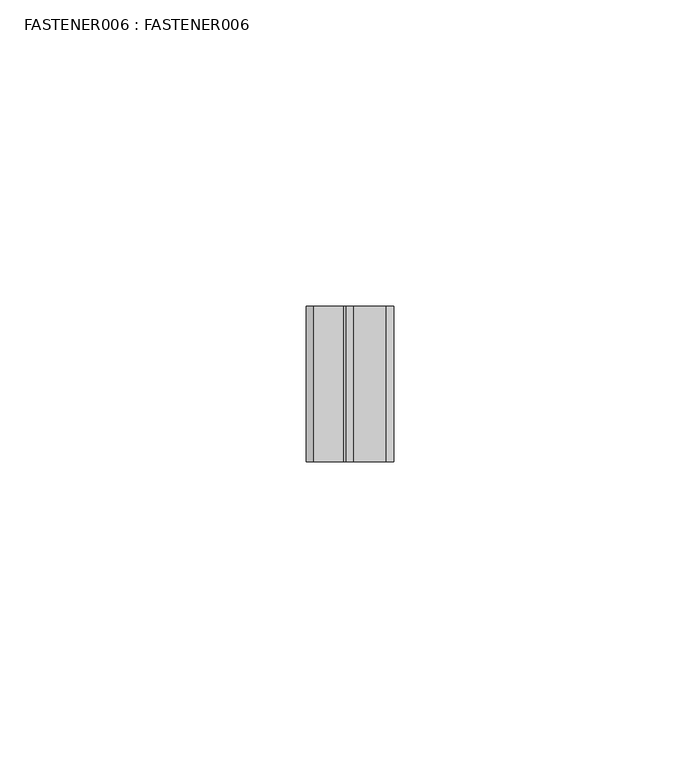
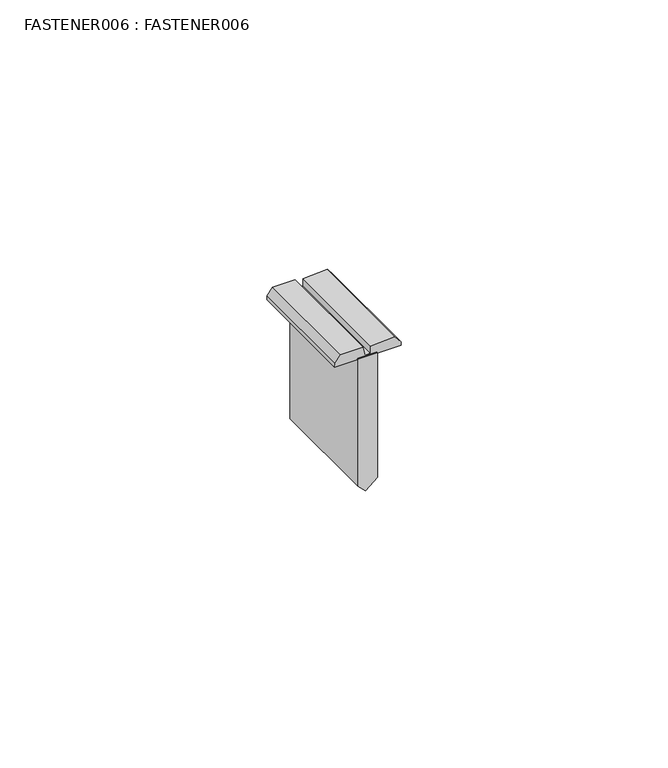
"""IFC4 building model written with IfcOpenShell, lengths in millimetres: proxy geometry, FASTENER006 : FASTENER006."""

from ifc_helpers import new_model, si_unit, frame, origin, place, context, project, spatial, polyline, outline, extrude, source, transform, mapped, element, save


def fastener006_fastener006_f031ca55(model_context):
    return source(origin(), model_context, "Body", "SweptSolid", [
        extrude(outline(polyline([(42577.1576024, 5870.6890035), (42548.1988623, 5870.6890035), (42546.5833096, 5872.3460181), (42548.7638676, 5874.895922), (42577.1576024, 5874.895922), (42577.1576024, 5870.6890035)])), frame((0.0, -1078.2906574, 0.0), z_axis=(0.0, 1.0, 0.0), x_axis=(0.0, 0.0, 1.0)), (0.0, 0.0, 1.0), 25.4),
        extrude(outline(polyline([(42577.1576024, 5879.9417891), (42577.9674245, 5879.9417891), (42579.5612959, 5878.7030871), (42579.1650604, 5873.4174049), (42577.5756297, 5873.4174049), (42577.5756297, 5872.1703), (42579.587761, 5871.7740645), (42579.587761, 5866.8949826), (42577.9938896, 5865.6562805), (42577.1576024, 5865.6454839), (42577.1576024, 5879.9417891)])), frame((0.0, -1078.2906574, 0.0), z_axis=(0.0, 1.0, 0.0), x_axis=(0.0, 0.0, 1.0)), (0.0, 0.0, 1.0), 25.4),
    ])


if __name__ == "__main__":
    model = new_model("IFC4")
    model_context = context("Model", 3, world=origin())
    ifc_project = project(units=[si_unit("LENGTHUNIT", "METRE", prefix="MILLI")], contexts=[model_context])
    site = spatial("IfcSite", under=ifc_project)
    building = spatial("IfcBuilding", under=site)
    placement = place(None, origin())
    fastener006_fastener006_shape = fastener006_fastener006_f031ca55(model_context)
    element("IfcBuildingElementProxy", 1, Name="FASTENER006 : FASTENER006", ObjectType="FASTENER006 : FASTENER006", at=placement, inside=building, context=model_context, shape_type="MappedRepresentation", body=[
        mapped(fastener006_fastener006_shape, transform((0.0, 0.0, 0.0), x_axis=(1.0, 0.0, 0.0), y_axis=(0.0, 1.0, 0.0), z_axis=(0.0, 0.0, 1.0))),
    ])
    save(model, "model.ifc")

# Revit data of these elements
# Type "FASTENER006 : FASTENER006"
#   NameOverride = "FASTENER006"
# Element 1 (IfcBuildingElementProxy, "FASTENER006 : FASTENER006")
#   Materials on its faces: "ENGINEERED PANCAKE HEAD FASTENER @ 12\" O.C."
# Materials
#   "ENGINEERED PANCAKE HEAD FASTENER @ 12\" O.C.": class "Unassigned", colour RGB 255 255 255, transparency 0, Cost = 0
